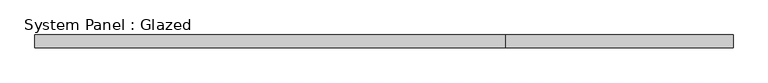
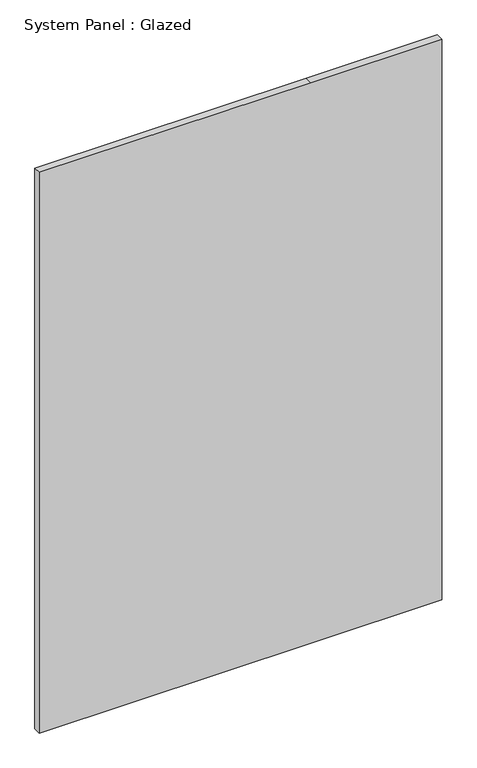
"""IFC4 building model written with IfcOpenShell, lengths in millimetres: plate geometry, System Panel : Glazed."""

import ifcopenshell
import ifcopenshell.guid

model = None  # the IFC model being written
_history = None  # IfcOwnerHistory: only IFC2X3 demands one
_inside = {}  # id of a spatial element -> (the spatial element, [elements in it])
_under = {}  # id of a project, library or spatial element -> (it, [spatial elements below it])
_declared = {}  # id of a project -> (the project, [libraries it declares])
_typed = {}  # id of a type object -> (the type object, [elements of that type])
_made_of = {}  # id of a material, layer set ... -> (it, [elements and type objects made of it])


def new_model(schema):
    """Start an empty IFC model of exactly this schema.

    Asked for "IFC4X3", IfcOpenShell would pick the latest addendum, in which some entities
    have other attributes; the version numbers below select the first issue.
    IFC2X3 requires an IfcOwnerHistory on every rooted entity: one is made here for all.
    """
    global model, _history
    if schema == "IFC4X3":
        model = ifcopenshell.file(schema_version=(4, 3, 0, 0))
    else:
        model = ifcopenshell.file(schema=schema)
    _inside.clear()
    _under.clear()
    _declared.clear()
    _typed.clear()
    _made_of.clear()
    _history = None
    if model.schema == "IFC2X3":
        org = make("IfcOrganization", Name="unknown")
        user = make(
            "IfcPersonAndOrganization",
            ThePerson=make("IfcPerson", FamilyName="unknown"),
            TheOrganization=org,
        )
        app = make(
            "IfcApplication",
            ApplicationDeveloper=org,
            Version="unknown",
            ApplicationFullName="unknown",
            ApplicationIdentifier="unknown",
        )
        _history = make(
            "IfcOwnerHistory",
            OwningUser=user,
            OwningApplication=app,
            ChangeAction="ADDED",
            CreationDate=0,
        )
    return model


def make(cls, **values):
    """One entity of the class cls with the attributes given. An attribute that is None is left unset."""
    return model.create_entity(
        cls, **{name: value for name, value in values.items() if value is not None}
    )


def rooted(cls, **values):
    """An entity with a GlobalId (a new one), such as an element, a storey or a relation."""
    return make(cls, GlobalId=ifcopenshell.guid.new(), OwnerHistory=_history, **values)


def si_unit(unit_type, name, prefix=None):
    """IfcSIUnit, for example si_unit("LENGTHUNIT", "METRE", prefix="MILLI")."""
    return make("IfcSIUnit", UnitType=unit_type, Prefix=prefix, Name=name)


def assignment(units):
    """IfcUnitAssignment: the units of a project."""
    return None if units is None else make("IfcUnitAssignment", Units=units)


def point(xyz):
    """IfcCartesianPoint."""
    return None if xyz is None else make("IfcCartesianPoint", Coordinates=xyz)


def direction(xyz):
    """IfcDirection."""
    return None if xyz is None else make("IfcDirection", DirectionRatios=xyz)


def frame(location, z_axis=None, x_axis=None):
    """IfcAxis2Placement3D, a coordinate frame: its origin and axes. An axis left out is left unset."""
    return make(
        "IfcAxis2Placement3D",
        Location=point(location),
        Axis=direction(z_axis),
        RefDirection=direction(x_axis),
    )


def origin():
    """The frame at (0, 0, 0) with its axes left unset."""
    return frame((0.0, 0.0, 0.0))


def place(relative_to, where):
    """IfcLocalPlacement: puts the frame where relative to a parent placement (None: the world)."""
    return make(
        "IfcLocalPlacement", PlacementRelTo=relative_to, RelativePlacement=where
    )


def context(
    kind, dimensions, precision=None, world=None, true_north=None, identifier=None
):
    """IfcGeometricRepresentationContext, for example the 3D "Model" context."""
    return make(
        "IfcGeometricRepresentationContext",
        ContextIdentifier=identifier,
        ContextType=kind,
        CoordinateSpaceDimension=dimensions,
        Precision=precision,
        WorldCoordinateSystem=world,
        TrueNorth=true_north,
    )


def project(units=None, contexts=None):
    """IfcProject with its units and contexts."""
    return rooted(
        "IfcProject",
        Name="project",
        RepresentationContexts=contexts,
        UnitsInContext=assignment(units),
    )


def spatial(cls, under=None, at=None, **own):
    """A site, building, storey or space (cls), placed at a placement, below another one or the project."""
    s = rooted(cls, ObjectPlacement=at, **own)
    if under is not None:
        _under.setdefault(under.id(), (under, []))[1].append(s)
    return s


def polyline(points):
    """IfcPolyline through the points."""
    return make("IfcPolyline", Points=[point(p) for p in points])


def outline(outer, holes=None, kind="AREA"):
    """IfcArbitraryClosedProfileDef: a profile drawn as a closed curve; with holes, ...WithVoids."""
    if holes is None:
        return make("IfcArbitraryClosedProfileDef", ProfileType=kind, OuterCurve=outer)
    return make(
        "IfcArbitraryProfileDefWithVoids",
        ProfileType=kind,
        OuterCurve=outer,
        InnerCurves=holes,
    )


def extrude(swept, where, along, depth):
    """IfcExtrudedAreaSolid: the profile swept, set in the frame where, extruded along a direction by depth."""
    return make(
        "IfcExtrudedAreaSolid",
        SweptArea=swept,
        Position=where,
        ExtrudedDirection=direction(along),
        Depth=depth,
    )


def shape(context_of_items, identifier, shape_type, items):
    """IfcShapeRepresentation: the items that make up one representation, for example the "Body"."""
    return make(
        "IfcShapeRepresentation",
        ContextOfItems=context_of_items,
        RepresentationIdentifier=identifier,
        RepresentationType=shape_type,
        Items=items,
    )


def source(mapping_origin, context_of_items, identifier, shape_type, items):
    """IfcRepresentationMap: a shape defined once, which mapped items show again and again."""
    return make(
        "IfcRepresentationMap",
        MappingOrigin=mapping_origin,
        MappedRepresentation=shape(context_of_items, identifier, shape_type, items),
    )


def transform(
    local_origin,
    x_axis=None,
    y_axis=None,
    z_axis=None,
    scale=None,
    scale2=None,
    scale3=None,
    uniform=True,
):
    """IfcCartesianTransformationOperator3D, or its non-uniform kind. x_axis, y_axis, z_axis: its Axis1, 2, 3."""
    if uniform:
        return make(
            "IfcCartesianTransformationOperator3D",
            Axis1=direction(x_axis),
            Axis2=direction(y_axis),
            LocalOrigin=point(local_origin),
            Scale=scale,
            Axis3=direction(z_axis),
        )
    return make(
        "IfcCartesianTransformationOperator3DnonUniform",
        Axis1=direction(x_axis),
        Axis2=direction(y_axis),
        LocalOrigin=point(local_origin),
        Scale=scale,
        Axis3=direction(z_axis),
        Scale2=scale2,
        Scale3=scale3,
    )


def mapped(mapping_source, mapping_target):
    """IfcMappedItem: shows the shape of a source again, moved by a transform."""
    return make(
        "IfcMappedItem", MappingSource=mapping_source, MappingTarget=mapping_target
    )


def made_of(thing, what):
    """Note that an element or type object is made of a material, layer set ...; save() writes the relation."""
    if what is not None:
        _made_of.setdefault(what.id(), (what, []))[1].append(thing)
    return thing


def element(
    cls,
    number,
    at=None,
    inside=None,
    cuts=None,
    type_object=None,
    material=None,
    context=None,
    identifier="Body",
    shape_type=None,
    held_by="IfcProductDefinitionShape",
    body=None,
    shapes=None,
    **own,
):
    """One element of the class cls, such as IfcWall. Its Tag is "e" and its number.

    at: its placement. inside: the storey or other place that contains it. cuts: it is an
    opening in that element (IfcRelVoidsElement). A single representation is given by context,
    identifier, shape_type and body (its items); several are given by shapes. held_by: the class
    of the entity that holds the representations. save() writes the other relations.
    """
    e = rooted(cls, Tag="e%d" % number, ObjectPlacement=at, **own)
    if body is not None:
        shapes = [shape(context, identifier, shape_type, body)]
    if shapes is not None:
        e.Representation = make(held_by, Representations=shapes)
    if inside is not None:
        _inside.setdefault(inside.id(), (inside, []))[1].append(e)
    if cuts is not None:
        rooted(
            "IfcRelVoidsElement", RelatingBuildingElement=cuts, RelatedOpeningElement=e
        )
    if type_object is not None:
        _typed.setdefault(type_object.id(), (type_object, []))[1].append(e)
    return made_of(e, material)


def aggregate(whole, parts):
    """IfcRelAggregates: a whole, such as a stair, and the parts it consists of."""
    return rooted("IfcRelAggregates", RelatingObject=whole, RelatedObjects=parts)


def save(model, path):
    """Write the relations noted so far, then the file.

    IfcRelAggregates (storeys below a building ...), IfcRelContainedInSpatialStructure (elements
    in a storey), IfcRelDefinesByType, IfcRelAssociatesMaterial and IfcRelDeclares: one each for
    every whole, place, type object, material and project.
    """
    for whole, parts in _under.values():
        aggregate(whole, parts)
    for where, things in _inside.values():
        rooted(
            "IfcRelContainedInSpatialStructure",
            RelatedElements=things,
            RelatingStructure=where,
        )
    for kind, things in _typed.values():
        rooted("IfcRelDefinesByType", RelatedObjects=things, RelatingType=kind)
    for what, things in _made_of.values():
        rooted("IfcRelAssociatesMaterial", RelatedObjects=things, RelatingMaterial=what)
    for by, libraries in _declared.values():
        rooted("IfcRelDeclares", RelatingContext=by, RelatedDefinitions=libraries)
    model.write(path)


def system_panel_glazed_b2aaa3aa(model_context):
    return source(origin(), model_context, "Body", "SweptSolid", [
        extrude(outline(polyline([(0.0, -692.15), (0.0, 241.3), (0.0, 692.15), (2038.35, 692.15), (2038.35, 241.3), (2038.35, -692.15), (0.0, -692.15)])), frame((0.0, -44.45, 0.0), z_axis=(0.0, 1.0, 0.0), x_axis=(0.0, 0.0, 1.0)), (0.0, 0.0, 1.0), 25.4),
    ])


if __name__ == "__main__":
    model = new_model("IFC4")
    model_context = context("Model", 3, world=origin())
    ifc_project = project(units=[si_unit("LENGTHUNIT", "METRE", prefix="MILLI")], contexts=[model_context])
    site = spatial("IfcSite", under=ifc_project)
    building = spatial("IfcBuilding", under=site)
    placement = place(None, origin())
    system_panel_glazed_shape = system_panel_glazed_b2aaa3aa(model_context)
    element("IfcPlate", 1, ObjectType="System Panel : Glazed", at=placement, inside=building, context=model_context, shape_type="MappedRepresentation", body=[
        mapped(system_panel_glazed_shape, transform((0.0, 0.0, 0.0), x_axis=(1.0, 0.0, 0.0), y_axis=(0.0, 1.0, 0.0), z_axis=(0.0, 0.0, 1.0))),
    ])
    save(model, "model.ifc")

# Revit data of these elements
# Project information
#   Project Issue Date = "Issue Date"
#   Project Status = "Project Status"
#   Client Name = "Owner"
#   Project Address = "Enter address here"
#   Project Name = "Project Name"
#   Project Number = "Project Number"
# Type "System Panel : Glazed"
#   Construction Type Id = "GSP4R"
#   Analytic Construction = "1/8 in Pilkington single glazing"
#   Visual Light Transmittance = 0.9
#   Solar Heat Gain Coefficient = 0.86
#   Heat Transfer Coefficient (U) = 1.18115 BTU/(h·ft²·°F)
#   Define Thermal Properties by = 1
# Element 1 (IfcPlate, "System Panel : Glazed")
#   Materials on its faces: "Glass"
# Materials
#   "Glass": class "Glass", colour RGB 0 0 255, transparency 0.75, Description = "Soda Lime Glass", Cost = 0
